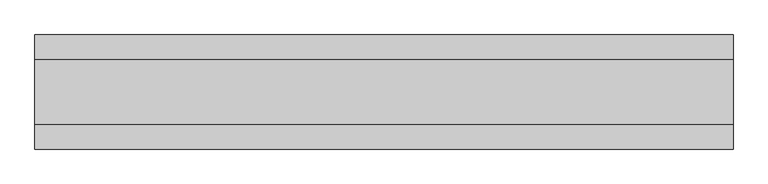
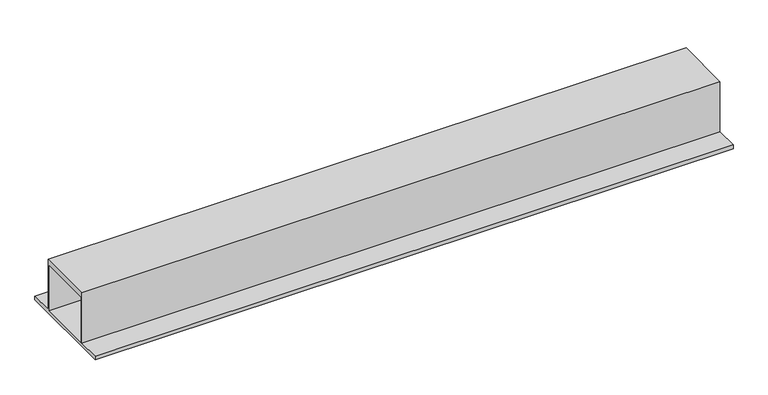
"""IFC4 building model written with IfcOpenShell, lengths in millimetres: beam geometry, NLRS_28_SF_LIB_stalen ligger THQ-AV-CWV-MMBS-SRP_gen_rsf : stalen ligger_gen__THQ_280x10-290x30-550x20."""

import ifcopenshell
import ifcopenshell.guid

model = None  # the IFC model being written
_history = None  # IfcOwnerHistory: only IFC2X3 demands one
_inside = {}  # id of a spatial element -> (the spatial element, [elements in it])
_under = {}  # id of a project, library or spatial element -> (it, [spatial elements below it])
_declared = {}  # id of a project -> (the project, [libraries it declares])
_typed = {}  # id of a type object -> (the type object, [elements of that type])
_made_of = {}  # id of a material, layer set ... -> (it, [elements and type objects made of it])


def new_model(schema):
    """Start an empty IFC model of exactly this schema.

    Asked for "IFC4X3", IfcOpenShell would pick the latest addendum, in which some entities
    have other attributes; the version numbers below select the first issue.
    IFC2X3 requires an IfcOwnerHistory on every rooted entity: one is made here for all.
    """
    global model, _history
    if schema == "IFC4X3":
        model = ifcopenshell.file(schema_version=(4, 3, 0, 0))
    else:
        model = ifcopenshell.file(schema=schema)
    _inside.clear()
    _under.clear()
    _declared.clear()
    _typed.clear()
    _made_of.clear()
    _history = None
    if model.schema == "IFC2X3":
        org = make("IfcOrganization", Name="unknown")
        user = make(
            "IfcPersonAndOrganization",
            ThePerson=make("IfcPerson", FamilyName="unknown"),
            TheOrganization=org,
        )
        app = make(
            "IfcApplication",
            ApplicationDeveloper=org,
            Version="unknown",
            ApplicationFullName="unknown",
            ApplicationIdentifier="unknown",
        )
        _history = make(
            "IfcOwnerHistory",
            OwningUser=user,
            OwningApplication=app,
            ChangeAction="ADDED",
            CreationDate=0,
        )
    return model


def make(cls, **values):
    """One entity of the class cls with the attributes given. An attribute that is None is left unset."""
    return model.create_entity(
        cls, **{name: value for name, value in values.items() if value is not None}
    )


def rooted(cls, **values):
    """An entity with a GlobalId (a new one), such as an element, a storey or a relation."""
    return make(cls, GlobalId=ifcopenshell.guid.new(), OwnerHistory=_history, **values)


def si_unit(unit_type, name, prefix=None):
    """IfcSIUnit, for example si_unit("LENGTHUNIT", "METRE", prefix="MILLI")."""
    return make("IfcSIUnit", UnitType=unit_type, Prefix=prefix, Name=name)


def assignment(units):
    """IfcUnitAssignment: the units of a project."""
    return None if units is None else make("IfcUnitAssignment", Units=units)


def point(xyz):
    """IfcCartesianPoint."""
    return None if xyz is None else make("IfcCartesianPoint", Coordinates=xyz)


def direction(xyz):
    """IfcDirection."""
    return None if xyz is None else make("IfcDirection", DirectionRatios=xyz)


def frame(location, z_axis=None, x_axis=None):
    """IfcAxis2Placement3D, a coordinate frame: its origin and axes. An axis left out is left unset."""
    return make(
        "IfcAxis2Placement3D",
        Location=point(location),
        Axis=direction(z_axis),
        RefDirection=direction(x_axis),
    )


def origin():
    """The frame at (0, 0, 0) with its axes left unset."""
    return frame((0.0, 0.0, 0.0))


def place(relative_to, where):
    """IfcLocalPlacement: puts the frame where relative to a parent placement (None: the world)."""
    return make(
        "IfcLocalPlacement", PlacementRelTo=relative_to, RelativePlacement=where
    )


def context(
    kind, dimensions, precision=None, world=None, true_north=None, identifier=None
):
    """IfcGeometricRepresentationContext, for example the 3D "Model" context."""
    return make(
        "IfcGeometricRepresentationContext",
        ContextIdentifier=identifier,
        ContextType=kind,
        CoordinateSpaceDimension=dimensions,
        Precision=precision,
        WorldCoordinateSystem=world,
        TrueNorth=true_north,
    )


def project(units=None, contexts=None):
    """IfcProject with its units and contexts."""
    return rooted(
        "IfcProject",
        Name="project",
        RepresentationContexts=contexts,
        UnitsInContext=assignment(units),
    )


def spatial(cls, under=None, at=None, **own):
    """A site, building, storey or space (cls), placed at a placement, below another one or the project."""
    s = rooted(cls, ObjectPlacement=at, **own)
    if under is not None:
        _under.setdefault(under.id(), (under, []))[1].append(s)
    return s


def polyline(points):
    """IfcPolyline through the points."""
    return make("IfcPolyline", Points=[point(p) for p in points])


def outline(outer, holes=None, kind="AREA"):
    """IfcArbitraryClosedProfileDef: a profile drawn as a closed curve; with holes, ...WithVoids."""
    if holes is None:
        return make("IfcArbitraryClosedProfileDef", ProfileType=kind, OuterCurve=outer)
    return make(
        "IfcArbitraryProfileDefWithVoids",
        ProfileType=kind,
        OuterCurve=outer,
        InnerCurves=holes,
    )


def extrude(swept, where, along, depth):
    """IfcExtrudedAreaSolid: the profile swept, set in the frame where, extruded along a direction by depth."""
    return make(
        "IfcExtrudedAreaSolid",
        SweptArea=swept,
        Position=where,
        ExtrudedDirection=direction(along),
        Depth=depth,
    )


def shape(context_of_items, identifier, shape_type, items):
    """IfcShapeRepresentation: the items that make up one representation, for example the "Body"."""
    return make(
        "IfcShapeRepresentation",
        ContextOfItems=context_of_items,
        RepresentationIdentifier=identifier,
        RepresentationType=shape_type,
        Items=items,
    )


def source(mapping_origin, context_of_items, identifier, shape_type, items):
    """IfcRepresentationMap: a shape defined once, which mapped items show again and again."""
    return make(
        "IfcRepresentationMap",
        MappingOrigin=mapping_origin,
        MappedRepresentation=shape(context_of_items, identifier, shape_type, items),
    )


def transform(
    local_origin,
    x_axis=None,
    y_axis=None,
    z_axis=None,
    scale=None,
    scale2=None,
    scale3=None,
    uniform=True,
):
    """IfcCartesianTransformationOperator3D, or its non-uniform kind. x_axis, y_axis, z_axis: its Axis1, 2, 3."""
    if uniform:
        return make(
            "IfcCartesianTransformationOperator3D",
            Axis1=direction(x_axis),
            Axis2=direction(y_axis),
            LocalOrigin=point(local_origin),
            Scale=scale,
            Axis3=direction(z_axis),
        )
    return make(
        "IfcCartesianTransformationOperator3DnonUniform",
        Axis1=direction(x_axis),
        Axis2=direction(y_axis),
        LocalOrigin=point(local_origin),
        Scale=scale,
        Axis3=direction(z_axis),
        Scale2=scale2,
        Scale3=scale3,
    )


def mapped(mapping_source, mapping_target):
    """IfcMappedItem: shows the shape of a source again, moved by a transform."""
    return make(
        "IfcMappedItem", MappingSource=mapping_source, MappingTarget=mapping_target
    )


def made_of(thing, what):
    """Note that an element or type object is made of a material, layer set ...; save() writes the relation."""
    if what is not None:
        _made_of.setdefault(what.id(), (what, []))[1].append(thing)
    return thing


def element(
    cls,
    number,
    at=None,
    inside=None,
    cuts=None,
    type_object=None,
    material=None,
    context=None,
    identifier="Body",
    shape_type=None,
    held_by="IfcProductDefinitionShape",
    body=None,
    shapes=None,
    **own,
):
    """One element of the class cls, such as IfcWall. Its Tag is "e" and its number.

    at: its placement. inside: the storey or other place that contains it. cuts: it is an
    opening in that element (IfcRelVoidsElement). A single representation is given by context,
    identifier, shape_type and body (its items); several are given by shapes. held_by: the class
    of the entity that holds the representations. save() writes the other relations.
    """
    e = rooted(cls, Tag="e%d" % number, ObjectPlacement=at, **own)
    if body is not None:
        shapes = [shape(context, identifier, shape_type, body)]
    if shapes is not None:
        e.Representation = make(held_by, Representations=shapes)
    if inside is not None:
        _inside.setdefault(inside.id(), (inside, []))[1].append(e)
    if cuts is not None:
        rooted(
            "IfcRelVoidsElement", RelatingBuildingElement=cuts, RelatedOpeningElement=e
        )
    if type_object is not None:
        _typed.setdefault(type_object.id(), (type_object, []))[1].append(e)
    return made_of(e, material)


def aggregate(whole, parts):
    """IfcRelAggregates: a whole, such as a stair, and the parts it consists of."""
    return rooted("IfcRelAggregates", RelatingObject=whole, RelatedObjects=parts)


def save(model, path):
    """Write the relations noted so far, then the file.

    IfcRelAggregates (storeys below a building ...), IfcRelContainedInSpatialStructure (elements
    in a storey), IfcRelDefinesByType, IfcRelAssociatesMaterial and IfcRelDeclares: one each for
    every whole, place, type object, material and project.
    """
    for whole, parts in _under.values():
        aggregate(whole, parts)
    for where, things in _inside.values():
        rooted(
            "IfcRelContainedInSpatialStructure",
            RelatedElements=things,
            RelatingStructure=where,
        )
    for kind, things in _typed.values():
        rooted("IfcRelDefinesByType", RelatedObjects=things, RelatingType=kind)
    for what, things in _made_of.values():
        rooted("IfcRelAssociatesMaterial", RelatedObjects=things, RelatingMaterial=what)
    for by, libraries in _declared.values():
        rooted("IfcRelDeclares", RelatingContext=by, RelatedDefinitions=libraries)
    model.write(path)


def beam_09e22bfa(model_context):
    return source(origin(), model_context, "Body", "SweptSolid", [
        extrude(outline(polyline([(143.5, 280.0), (143.5, 0.0), (263.5, 0.0), (263.5, -20.0), (-286.5, -20.0), (-286.5, 0.0), (-166.5, 0.0), (-166.5, 280.0), (143.5, 280.0)]), holes=[polyline([(133.5, 0.0), (133.5, 250.0), (-156.5, 250.0), (-156.5, 0.0), (133.5, 0.0)])]), frame((-1682.5, 0.0, 0.0), z_axis=(1.0, 0.0, 0.0), x_axis=(0.0, 1.0, 0.0)), (0.0, 0.0, 1.0), 3365.0),
    ])


if __name__ == "__main__":
    model = new_model("IFC4")
    model_context = context("Model", 3, world=origin())
    ifc_project = project(units=[si_unit("LENGTHUNIT", "METRE", prefix="MILLI")], contexts=[model_context])
    site = spatial("IfcSite", under=ifc_project)
    building = spatial("IfcBuilding", under=site)
    placement = place(None, origin())
    beam_shape = beam_09e22bfa(model_context)
    element("IfcBeam", 1, ObjectType="NLRS_28_SF_LIB_stalen ligger THQ-AV-CWV-MMBS-SRP_gen_rsf : stalen ligger_gen__THQ_280x10-290x30-550x20", at=placement, inside=building, context=model_context, shape_type="MappedRepresentation", body=[
        mapped(beam_shape, transform((0.0, 0.0, 0.0), x_axis=(1.0, 0.0, 0.0), y_axis=(0.0, 1.0, 0.0), z_axis=(0.0, 0.0, 1.0))),
    ])
    save(model, "model.ifc")

# Revit data of these elements
# Type "NLRS_28_SF_LIB_stalen ligger THQ-AV-CWV-MMBS-SRP_gen_rsf : stalen ligger_gen__THQ_280x10-290x30-550x20"
#   Type IfcGUID = "2GRbcre991teoKeCLB8MAm"
#   IfcExportAs = "IfcBeamType"
#   Type Comments = "THQ 280x10-290x30-550x20"
#   Model = " "
#   Manufacturer = " "
#   Fire Rating = " "
#   Description = "stalen ligger THQ 280x10-290x30-550x20"
#   Assembly Code = "28.11"
#   tw = 10 mm
#   tu = 20 mm
#   to = 30 mm
#   h = 280 mm
#   bu = 550 mm
#   bo = 290 mm
#   NLRS_C_lengte [instance default] = 1500 mm
#   Length [instance default] = 1500 mm
#   RSF_C_vullen_met_beton [instance default] = no
#   RSF_C_petligger = no
#   RSF_C_hoedligger = yes
#   Structural Material = NLRS_h2_staal_gen_rsf
#   Keynote = ""
# Element 1 (IfcBeam, "NLRS_28_SF_LIB_stalen ligger THQ-AV-CWV-MMBS-SRP_gen_rsf : stalen ligger_gen__THQ_280x10-290x30-550x20")
#   NLRS_C_lengte = 3365 mm
#   Materials on its faces: "NLRS_h2_staal_gen_rsf"
# Materials
#   "NLRS_h2_staal_gen_rsf": class "H - Metaal", colour RGB 189 187 185, transparency 0, Keynote = "h2", Manufacturer = "Revit Standards Foundation", URL = "www.revitstandards.org", Description = "staal", Cost = 0
